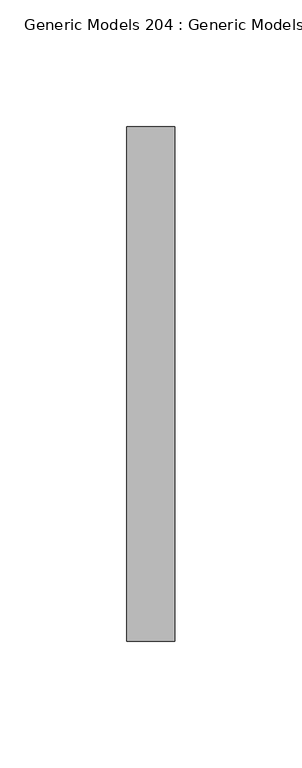
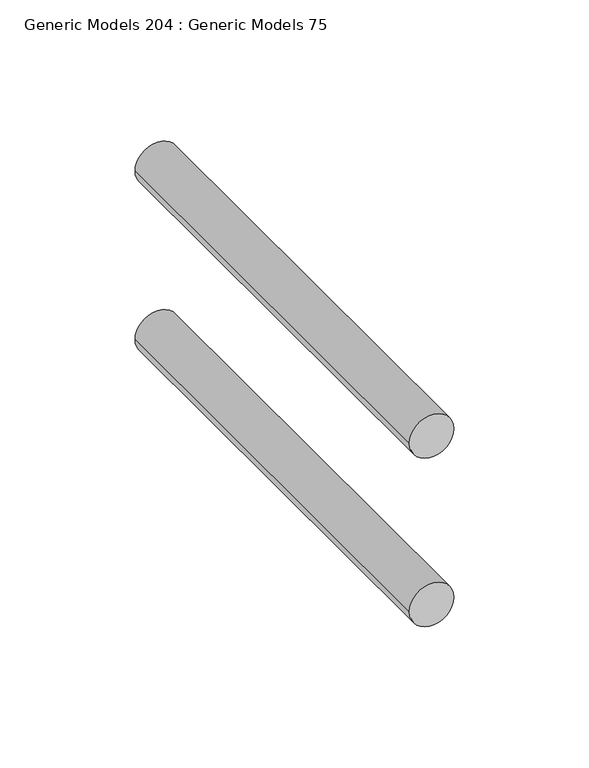
"""IFC4 building model written with IfcOpenShell, lengths in millimetres: proxy geometry, Generic Models 204 : Generic Models 75."""

from ifc_helpers import new_model, si_unit, point, frame, frame_2d, origin, place, context, project, spatial, circle_curve, trimmed, segment, composite_curve, outline, extrude, source, transform, mapped, element, save


def generic_models_204_generic_models_75_686e9af7(model_context):
    return source(origin(), model_context, "Body", "SweptSolid", [
        extrude(outline(composite_curve([segment(trimmed(circle_curve(frame_2d((271613.3125, 31975.4096032)), 9.525), [point((271613.3125, 31965.8846032))], [point((271613.3125, 31984.9346032))], False, "CARTESIAN"), True, "CONTINUOUS"), segment(trimmed(circle_curve(frame_2d((271613.3125, 31975.4096032)), 9.525), [point((271613.3125, 31984.9346032))], [point((271613.3125, 31965.8846032))], False, "CARTESIAN"), True, "CONTINUOUS")], self_intersect=False)), frame((0.0, 36305.8207942, 0.0), z_axis=(0.0, 1.0, 0.0), x_axis=(0.0, 0.0, 1.0)), (0.0, 0.0, 1.0), 203.2),
        extrude(outline(composite_curve([segment(trimmed(circle_curve(frame_2d((271689.5125, 31975.4096032)), 9.525), [point((271689.5125, 31965.8846032))], [point((271689.5125, 31984.9346032))], False, "CARTESIAN"), True, "CONTINUOUS"), segment(trimmed(circle_curve(frame_2d((271689.5125, 31975.4096032)), 9.525), [point((271689.5125, 31984.9346032))], [point((271689.5125, 31965.8846032))], False, "CARTESIAN"), True, "CONTINUOUS")], self_intersect=False)), frame((0.0, 36305.8207942, 0.0), z_axis=(0.0, 1.0, 0.0), x_axis=(0.0, 0.0, 1.0)), (0.0, 0.0, 1.0), 203.2),
    ])


if __name__ == "__main__":
    model = new_model("IFC4")
    model_context = context("Model", 3, world=origin())
    ifc_project = project(units=[si_unit("LENGTHUNIT", "METRE", prefix="MILLI")], contexts=[model_context])
    site = spatial("IfcSite", under=ifc_project)
    building = spatial("IfcBuilding", under=site)
    placement = place(None, origin())
    generic_models_204_generic_models_75_shape = generic_models_204_generic_models_75_686e9af7(model_context)
    element("IfcBuildingElementProxy", 1, Name="Generic Models 204 : Generic Models 75", ObjectType="Generic Models 204 : Generic Models 75", at=placement, inside=building, context=model_context, shape_type="MappedRepresentation", body=[
        mapped(generic_models_204_generic_models_75_shape, transform((0.0, 0.0, 0.0), x_axis=(1.0, 0.0, 0.0), y_axis=(0.0, 1.0, 0.0), z_axis=(0.0, 0.0, 1.0))),
    ])
    save(model, "model.ifc")
